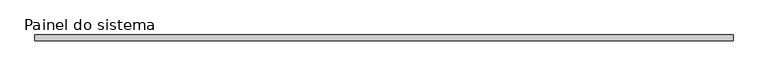
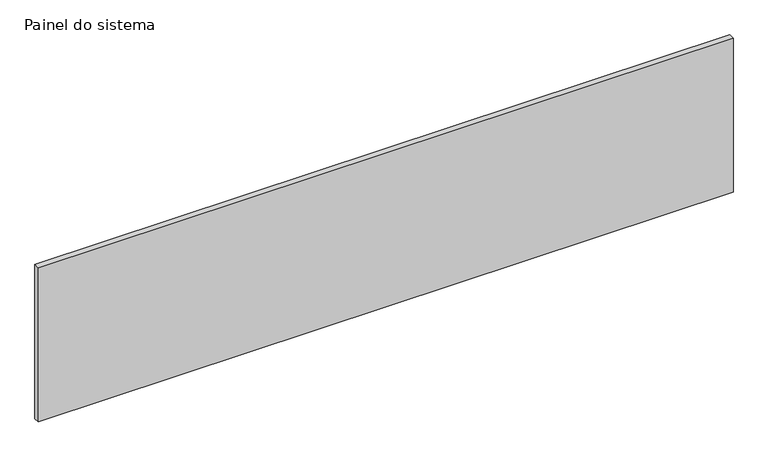
"""IFC4 building model written with IfcOpenShell, lengths in millimetres: plate geometry, Painel do sistema : Envidraçado."""

from ifc_helpers import new_model, si_unit, origin, origin_with_axes, place, context, project, spatial, polyline, outline, extrude, source, transform, mapped, element, save


def painel_do_sistema_7f6e6910(model_context):
    return source(origin(), model_context, "Body", "SweptSolid", [
        extrude(outline(polyline([(1462.4999925, 24.5), (-1462.4999925, 24.5), (-1462.4999925, 49.5), (1462.4999925, 49.5), (1462.4999925, 24.5)])), origin_with_axes(), (0.0, 0.0, 1.0), 685.7133319),
    ])


if __name__ == "__main__":
    model = new_model("IFC4")
    model_context = context("Model", 3, world=origin())
    ifc_project = project(units=[si_unit("LENGTHUNIT", "METRE", prefix="MILLI")], contexts=[model_context])
    site = spatial("IfcSite", under=ifc_project)
    building = spatial("IfcBuilding", under=site)
    placement = place(None, origin())
    painel_do_sistema_shape = painel_do_sistema_7f6e6910(model_context)
    element("IfcPlate", 1, ObjectType="Painel do sistema : Envidraçado", at=placement, inside=building, context=model_context, shape_type="MappedRepresentation", body=[
        mapped(painel_do_sistema_shape, transform((0.0, 0.0, 0.0), x_axis=(1.0, 0.0, 0.0), y_axis=(0.0, 1.0, 0.0), z_axis=(0.0, 0.0, 1.0))),
    ])
    save(model, "model.ifc")

# Revit data of these elements
# Type "Painel do sistema : Envidraçado"
#   Construction Type Id = "GSP4R"
#   Analytic Construction = "Vidraça única Pilkington 1/8 pol"
#   Visual Light Transmittance = 0.9
#   Solar Heat Gain Coefficient = 0.86
#   Heat Transfer Coefficient (U) = 6.7069 W/(m²·K)
# Element 1 (IfcPlate, "Painel do sistema : Envidraçado")
#   Materials on its faces: "Vidro"
# Materials
#   "Vidro": class "Vidro", colour RGB 0 128 192, transparency 0.9, Description = "Vidro de sílica", Cost = 0
